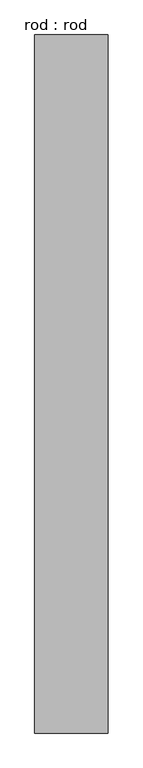
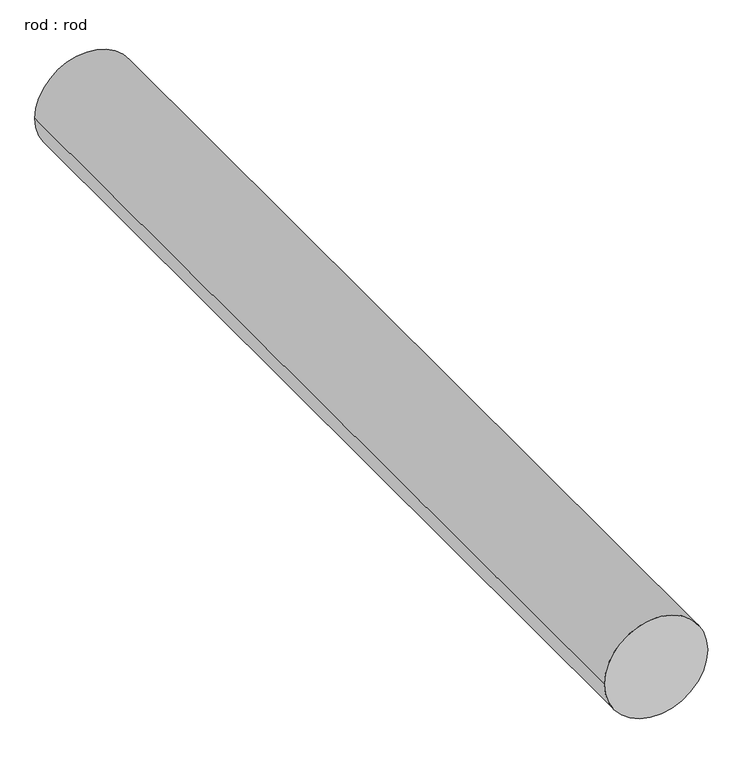
"""IFC4 building model written with IfcOpenShell, lengths in millimetres: proxy geometry, rod : rod."""

from ifc_helpers import new_model, si_unit, point, frame, frame_2d, origin, place, context, project, spatial, circle_curve, trimmed, segment, composite_curve, outline, extrude, source, transform, mapped, element, save


def rod_rod_12a53658(model_context):
    return source(origin(), model_context, "Body", "SweptSolid", [
        extrude(outline(composite_curve([segment(trimmed(circle_curve(frame_2d((0.0108462, 0.0)), 200.0), [point((0.0108462, 200.0))], [point((0.0108462, -200.0))], False, "CARTESIAN"), True, "CONTINUOUS"), segment(trimmed(circle_curve(frame_2d((0.0108462, 0.0)), 200.0), [point((0.0108462, -200.0))], [point((0.0108462, 200.0))], False, "CARTESIAN"), True, "CONTINUOUS")], self_intersect=False)), frame((0.0, 2187.0118866, 0.0), z_axis=(0.0, 1.0, 0.0), x_axis=(0.0, 0.0, 1.0)), (0.0, 0.0, 1.0), 3811.4334574),
    ])


if __name__ == "__main__":
    model = new_model("IFC4")
    model_context = context("Model", 3, world=origin())
    ifc_project = project(units=[si_unit("LENGTHUNIT", "METRE", prefix="MILLI")], contexts=[model_context])
    site = spatial("IfcSite", under=ifc_project)
    building = spatial("IfcBuilding", under=site)
    placement = place(None, origin())
    rod_rod_shape = rod_rod_12a53658(model_context)
    element("IfcBuildingElementProxy", 1, Name="rod : rod", ObjectType="rod : rod", at=placement, inside=building, context=model_context, shape_type="MappedRepresentation", body=[
        mapped(rod_rod_shape, transform((0.0, 0.0, 0.0), x_axis=(1.0, 0.0, 0.0), y_axis=(0.0, 1.0, 0.0), z_axis=(0.0, 0.0, 1.0))),
    ])
    save(model, "model.ifc")

# Revit data of these elements
# Type "rod : rod"
#   Default Elevation = 0
